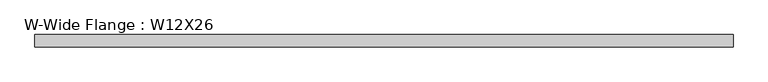
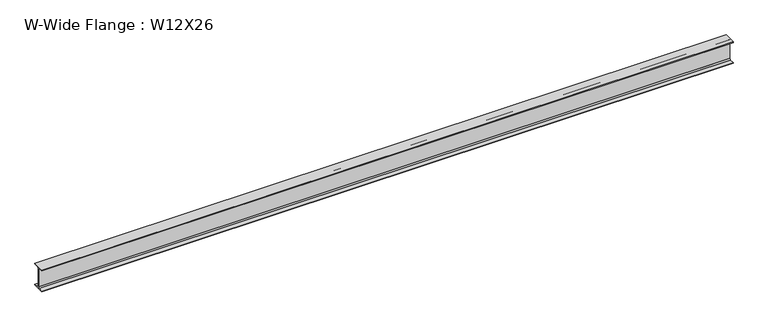
"""IFC4 building model written with IfcOpenShell, lengths in millimetres: beam geometry, W-Wide Flange : W12X26."""

from ifc_helpers import new_model, si_unit, point, frame, frame_2d, origin, place, context, project, spatial, polyline, circle_curve, trimmed, segment, composite_curve, outline, extrude, source, transform, mapped, element, save


def w_wide_flange_w12x26_ab3b7068(model_context):
    return source(origin(), model_context, "Body", "SweptSolid", [
        extrude(outline(composite_curve([segment(polyline([(82.423, -145.288), (82.423, -154.94), (-82.423, -154.94), (-82.423, -145.288), (-20.2565, -145.288)]), True, "CONTINUOUS"), segment(trimmed(circle_curve(frame_2d((-20.2565, -127.9525)), 17.3355), [point((-20.2565, -145.288))], [point((-2.921, -127.9525))], True, "CARTESIAN"), True, "CONTINUOUS"), segment(polyline([(-2.921, -127.9525), (-2.921, 127.9525)]), True, "CONTINUOUS"), segment(trimmed(circle_curve(frame_2d((-20.2565, 127.9525)), 17.3355), [point((-2.921, 127.9525))], [point((-20.2565, 145.288))], True, "CARTESIAN"), True, "CONTINUOUS"), segment(polyline([(-20.2565, 145.288), (-82.423, 145.288), (-82.423, 154.94), (82.423, 154.94), (82.423, 145.288), (20.2565, 145.288)]), True, "CONTINUOUS"), segment(trimmed(circle_curve(frame_2d((20.2565, 127.9525)), 17.3355), [point((20.2565, 145.288))], [point((2.921, 127.9525))], True, "CARTESIAN"), True, "CONTINUOUS"), segment(polyline([(2.921, 127.9525), (2.921, -127.9525)]), True, "CONTINUOUS"), segment(trimmed(circle_curve(frame_2d((20.2565, -127.9525)), 17.3355), [point((2.921, -127.9525))], [point((20.2565, -145.288))], True, "CARTESIAN"), True, "CONTINUOUS"), segment(polyline([(20.2565, -145.288), (82.423, -145.288)]), True, "CONTINUOUS")], self_intersect=False)), frame((-4749.8, 0.0, 0.0), z_axis=(1.0, 0.0, 0.0), x_axis=(0.0, 1.0, 0.0)), (0.0, 0.0, 1.0), 9429.5919799),
    ])


if __name__ == "__main__":
    model = new_model("IFC4")
    model_context = context("Model", 3, world=origin())
    ifc_project = project(units=[si_unit("LENGTHUNIT", "METRE", prefix="MILLI")], contexts=[model_context])
    site = spatial("IfcSite", under=ifc_project)
    building = spatial("IfcBuilding", under=site)
    placement = place(None, origin())
    w_wide_flange_w12x26_shape = w_wide_flange_w12x26_ab3b7068(model_context)
    element("IfcBeam", 1, ObjectType="W-Wide Flange : W12X26", at=placement, inside=building, context=model_context, shape_type="MappedRepresentation", body=[
        mapped(w_wide_flange_w12x26_shape, transform((0.0, 0.0, 0.0), x_axis=(1.0, 0.0, 0.0), y_axis=(0.0, 1.0, 0.0), z_axis=(0.0, 0.0, 1.0))),
    ])
    save(model, "model.ifc")

# Revit data of these elements
# Type "W-Wide Flange : W12X26"
#   Assembly Code = "B10"
#   W = 26
#   Length [instance default] = 5' - 0"
#   bf = 0' - 6.49"
#   d = 1' - 0.2"
#   k = 0' - 1 1/16"
#   k2 = 0' - 0.6825"
#   tf = 0' - 0.38"
#   tw = 0' - 0.23"
#   A = 0.053125 SF
#   Structural Material [instance default] = Steel ASTM A992
# Element 1 (IfcBeam, "W-Wide Flange : W12X26")
#   Materials on its faces: "Steel ASTM A992"
# Materials
#   "Steel ASTM A992": class "Metal", colour RGB 199 199 199, transparency 0, Description = "Structural steel 50ksi", Cost = 0
